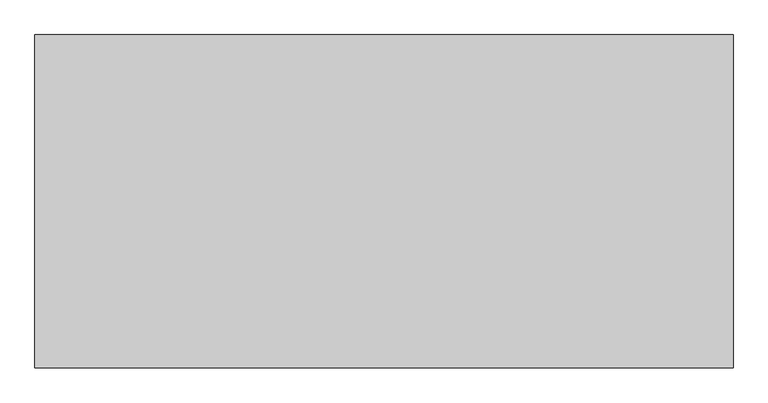
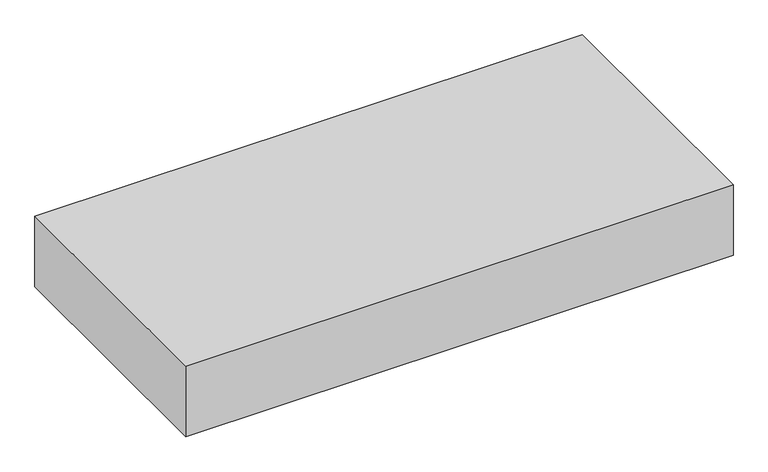
"""IFC4 building model written with IfcOpenShell, lengths in millimetres: proxy geometry, Space Planning Box_hec : Space Planning Box_hec."""

from ifc_helpers import new_model, si_unit, origin, origin_with_axes, place, context, project, spatial, polyline, outline, extrude, source, transform, mapped, element, save


def generic_models_7e8091d6(model_context):
    return source(origin(), model_context, "Body", "SweptSolid", [
        extrude(outline(polyline([(22000.0, 10500.0), (22000.0, -10500.0), (-22000.0, -10500.0), (-22000.0, 10500.0), (22000.0, 10500.0)])), origin_with_axes(), (0.0, 0.0, 1.0), 6000.0),
    ])


if __name__ == "__main__":
    model = new_model("IFC4")
    model_context = context("Model", 3, world=origin())
    ifc_project = project(units=[si_unit("LENGTHUNIT", "METRE", prefix="MILLI")], contexts=[model_context])
    site = spatial("IfcSite", under=ifc_project)
    building = spatial("IfcBuilding", under=site)
    placement = place(None, origin())
    generic_models_shape = generic_models_7e8091d6(model_context)
    element("IfcBuildingElementProxy", 1, Name="Space Planning Box_hec : Space Planning Box_hec", ObjectType="Space Planning Box_hec : Space Planning Box_hec", at=placement, inside=building, context=model_context, shape_type="MappedRepresentation", body=[
        mapped(generic_models_shape, transform((0.0, 0.0, 0.0), x_axis=(1.0, 0.0, 0.0), y_axis=(0.0, 1.0, 0.0), z_axis=(0.0, 0.0, 1.0))),
    ])
    save(model, "model.ifc")

# Revit data of these elements
# Type "Space Planning Box_hec : Space Planning Box_hec"
#   Type Comments = "..."
#   Room Name [instance default] = "?"
#   Interior Finish [instance default] = ""
#   Exterior Finish [instance default] = ""
#   Department [instance default] = ""
#   Assembly Code = "..."
#   Width [instance default] = 1524 mm
#   Program Area [instance default] = 0.00 m²
#   Length [instance default] = 1524 mm
#   Height [instance default] = 1524 mm
#   Area [instance default] = 2.32258 m²
#   Fill Color [instance default] = Cyan
#   Default Elevation = 0
# Element 1 (IfcBuildingElementProxy, "Space Planning Box_hec : Space Planning Box_hec")
#   Room Name = "Corridor"
#   Interior Finish = "IF2-1"
#   Exterior Finish = "EF1"
#   Department = "AR"
#   Width = 44000 mm
#   Length = 21000 mm
#   Height = 6000 mm
#   Area = 924.00 m²
#   Fill Color = Lavender
#   Materials on its faces: "Lavender"
# Materials
#   "Cyan": class "Generic", colour RGB 0 255 255, transparency 0.2, Cost = 0
#   "Lavender": class "Generic", colour RGB 186 85 211, transparency 0.2, Cost = 0
